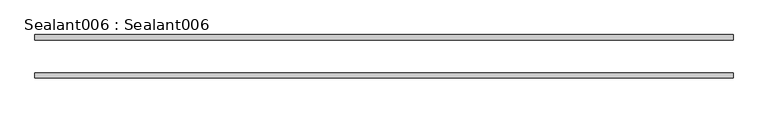
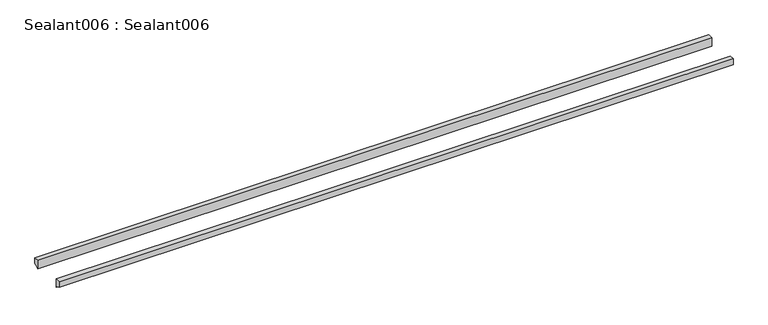
"""IFC4 building model written with IfcOpenShell, lengths in millimetres: proxy geometry, Sealant006 : Sealant006."""

from ifc_helpers import new_model, si_unit, point, frame, frame_2d, origin, place, context, project, spatial, polyline, circle_curve, trimmed, segment, composite_curve, outline, extrude, source, transform, mapped, element, save


def sealant006_sealant006_b0616daf(model_context):
    return source(origin(), model_context, "Body", "SweptSolid", [
        extrude(outline(composite_curve([segment(polyline([(9625.2926199, 39526.7507088), (9625.2926199, 39552.896), (9640.2075717, 39552.896), (9640.2075717, 39534.7027575)]), True, "CONTINUOUS"), segment(trimmed(circle_curve(frame_2d((9644.4481724, 39508.7856894)), 26.2617043), [point((9640.2075717, 39534.7027575))], [point((9625.2926199, 39526.7507088))], True, "CARTESIAN"), True, "CONTINUOUS")], self_intersect=False)), frame((-9232.0719278, 0.0, 0.0), z_axis=(1.0, 0.0, 0.0), x_axis=(0.0, 1.0, 0.0)), (0.0, 0.0, 1.0), 1999.85),
        extrude(outline(composite_curve([segment(trimmed(circle_curve(frame_2d((9511.3767366, 39508.7856894)), 26.2617043), [point((9530.5322891, 39526.7507088))], [point((9515.6173373, 39534.7027575))], True, "CARTESIAN"), True, "CONTINUOUS"), segment(polyline([(9515.6173373, 39534.7027575), (9515.6173373, 39552.896), (9530.5322891, 39552.896), (9530.5322891, 39526.7507088)]), True, "CONTINUOUS")], self_intersect=False)), frame((-9232.0719278, 0.0, 0.0), z_axis=(1.0, 0.0, 0.0), x_axis=(0.0, 1.0, 0.0)), (0.0, 0.0, 1.0), 1999.85),
    ])


if __name__ == "__main__":
    model = new_model("IFC4")
    model_context = context("Model", 3, world=origin())
    ifc_project = project(units=[si_unit("LENGTHUNIT", "METRE", prefix="MILLI")], contexts=[model_context])
    site = spatial("IfcSite", under=ifc_project)
    building = spatial("IfcBuilding", under=site)
    placement = place(None, origin())
    sealant006_sealant006_shape = sealant006_sealant006_b0616daf(model_context)
    element("IfcBuildingElementProxy", 1, Name="Sealant006 : Sealant006", ObjectType="Sealant006 : Sealant006", at=placement, inside=building, context=model_context, shape_type="MappedRepresentation", body=[
        mapped(sealant006_sealant006_shape, transform((0.0, 0.0, 0.0), x_axis=(1.0, 0.0, 0.0), y_axis=(0.0, 1.0, 0.0), z_axis=(0.0, 0.0, 1.0))),
    ])
    save(model, "model.ifc")

# Revit data of these elements
# Type "Sealant006 : Sealant006"
#   NameOverride = "Sealant006"
# Element 1 (IfcBuildingElementProxy, "Sealant006 : Sealant006")
#   Materials on its faces: "SEALANT AND BACKER ROD WHERE NECESSARY"
# Materials
#   "SEALANT AND BACKER ROD WHERE NECESSARY": class "Unassigned", colour RGB 225 240 198, transparency 0, Cost = 0
